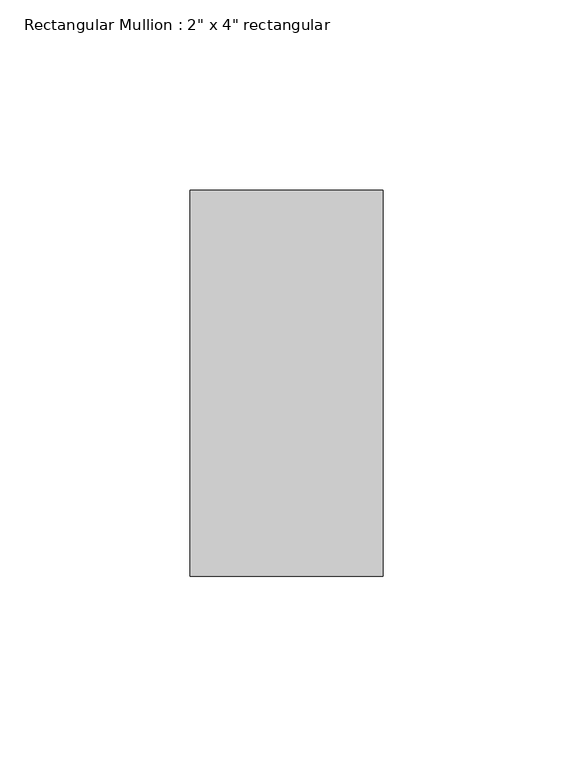
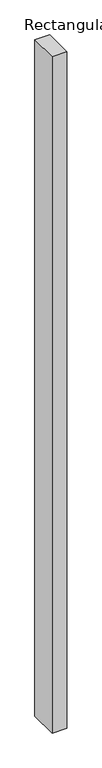
"""IFC4 building model written with IfcOpenShell, lengths in millimetres: member geometry."""

import ifcopenshell
import ifcopenshell.guid

model = None  # the IFC model being written
_history = None  # IfcOwnerHistory: only IFC2X3 demands one
_inside = {}  # id of a spatial element -> (the spatial element, [elements in it])
_under = {}  # id of a project, library or spatial element -> (it, [spatial elements below it])
_declared = {}  # id of a project -> (the project, [libraries it declares])
_typed = {}  # id of a type object -> (the type object, [elements of that type])
_made_of = {}  # id of a material, layer set ... -> (it, [elements and type objects made of it])


def new_model(schema):
    """Start an empty IFC model of exactly this schema.

    Asked for "IFC4X3", IfcOpenShell would pick the latest addendum, in which some entities
    have other attributes; the version numbers below select the first issue.
    IFC2X3 requires an IfcOwnerHistory on every rooted entity: one is made here for all.
    """
    global model, _history
    if schema == "IFC4X3":
        model = ifcopenshell.file(schema_version=(4, 3, 0, 0))
    else:
        model = ifcopenshell.file(schema=schema)
    _inside.clear()
    _under.clear()
    _declared.clear()
    _typed.clear()
    _made_of.clear()
    _history = None
    if model.schema == "IFC2X3":
        org = make("IfcOrganization", Name="unknown")
        user = make(
            "IfcPersonAndOrganization",
            ThePerson=make("IfcPerson", FamilyName="unknown"),
            TheOrganization=org,
        )
        app = make(
            "IfcApplication",
            ApplicationDeveloper=org,
            Version="unknown",
            ApplicationFullName="unknown",
            ApplicationIdentifier="unknown",
        )
        _history = make(
            "IfcOwnerHistory",
            OwningUser=user,
            OwningApplication=app,
            ChangeAction="ADDED",
            CreationDate=0,
        )
    return model


def make(cls, **values):
    """One entity of the class cls with the attributes given. An attribute that is None is left unset."""
    return model.create_entity(
        cls, **{name: value for name, value in values.items() if value is not None}
    )


def rooted(cls, **values):
    """An entity with a GlobalId (a new one), such as an element, a storey or a relation."""
    return make(cls, GlobalId=ifcopenshell.guid.new(), OwnerHistory=_history, **values)


def si_unit(unit_type, name, prefix=None):
    """IfcSIUnit, for example si_unit("LENGTHUNIT", "METRE", prefix="MILLI")."""
    return make("IfcSIUnit", UnitType=unit_type, Prefix=prefix, Name=name)


def assignment(units):
    """IfcUnitAssignment: the units of a project."""
    return None if units is None else make("IfcUnitAssignment", Units=units)


def point(xyz):
    """IfcCartesianPoint."""
    return None if xyz is None else make("IfcCartesianPoint", Coordinates=xyz)


def direction(xyz):
    """IfcDirection."""
    return None if xyz is None else make("IfcDirection", DirectionRatios=xyz)


def frame(location, z_axis=None, x_axis=None):
    """IfcAxis2Placement3D, a coordinate frame: its origin and axes. An axis left out is left unset."""
    return make(
        "IfcAxis2Placement3D",
        Location=point(location),
        Axis=direction(z_axis),
        RefDirection=direction(x_axis),
    )


def origin():
    """The frame at (0, 0, 0) with its axes left unset."""
    return frame((0.0, 0.0, 0.0))


def place(relative_to, where):
    """IfcLocalPlacement: puts the frame where relative to a parent placement (None: the world)."""
    return make(
        "IfcLocalPlacement", PlacementRelTo=relative_to, RelativePlacement=where
    )


def context(
    kind, dimensions, precision=None, world=None, true_north=None, identifier=None
):
    """IfcGeometricRepresentationContext, for example the 3D "Model" context."""
    return make(
        "IfcGeometricRepresentationContext",
        ContextIdentifier=identifier,
        ContextType=kind,
        CoordinateSpaceDimension=dimensions,
        Precision=precision,
        WorldCoordinateSystem=world,
        TrueNorth=true_north,
    )


def project(units=None, contexts=None):
    """IfcProject with its units and contexts."""
    return rooted(
        "IfcProject",
        Name="project",
        RepresentationContexts=contexts,
        UnitsInContext=assignment(units),
    )


def spatial(cls, under=None, at=None, **own):
    """A site, building, storey or space (cls), placed at a placement, below another one or the project."""
    s = rooted(cls, ObjectPlacement=at, **own)
    if under is not None:
        _under.setdefault(under.id(), (under, []))[1].append(s)
    return s


def polyline(points):
    """IfcPolyline through the points."""
    return make("IfcPolyline", Points=[point(p) for p in points])


def outline(outer, holes=None, kind="AREA"):
    """IfcArbitraryClosedProfileDef: a profile drawn as a closed curve; with holes, ...WithVoids."""
    if holes is None:
        return make("IfcArbitraryClosedProfileDef", ProfileType=kind, OuterCurve=outer)
    return make(
        "IfcArbitraryProfileDefWithVoids",
        ProfileType=kind,
        OuterCurve=outer,
        InnerCurves=holes,
    )


def extrude(swept, where, along, depth):
    """IfcExtrudedAreaSolid: the profile swept, set in the frame where, extruded along a direction by depth."""
    return make(
        "IfcExtrudedAreaSolid",
        SweptArea=swept,
        Position=where,
        ExtrudedDirection=direction(along),
        Depth=depth,
    )


def shape(context_of_items, identifier, shape_type, items):
    """IfcShapeRepresentation: the items that make up one representation, for example the "Body"."""
    return make(
        "IfcShapeRepresentation",
        ContextOfItems=context_of_items,
        RepresentationIdentifier=identifier,
        RepresentationType=shape_type,
        Items=items,
    )


def source(mapping_origin, context_of_items, identifier, shape_type, items):
    """IfcRepresentationMap: a shape defined once, which mapped items show again and again."""
    return make(
        "IfcRepresentationMap",
        MappingOrigin=mapping_origin,
        MappedRepresentation=shape(context_of_items, identifier, shape_type, items),
    )


def transform(
    local_origin,
    x_axis=None,
    y_axis=None,
    z_axis=None,
    scale=None,
    scale2=None,
    scale3=None,
    uniform=True,
):
    """IfcCartesianTransformationOperator3D, or its non-uniform kind. x_axis, y_axis, z_axis: its Axis1, 2, 3."""
    if uniform:
        return make(
            "IfcCartesianTransformationOperator3D",
            Axis1=direction(x_axis),
            Axis2=direction(y_axis),
            LocalOrigin=point(local_origin),
            Scale=scale,
            Axis3=direction(z_axis),
        )
    return make(
        "IfcCartesianTransformationOperator3DnonUniform",
        Axis1=direction(x_axis),
        Axis2=direction(y_axis),
        LocalOrigin=point(local_origin),
        Scale=scale,
        Axis3=direction(z_axis),
        Scale2=scale2,
        Scale3=scale3,
    )


def mapped(mapping_source, mapping_target):
    """IfcMappedItem: shows the shape of a source again, moved by a transform."""
    return make(
        "IfcMappedItem", MappingSource=mapping_source, MappingTarget=mapping_target
    )


def made_of(thing, what):
    """Note that an element or type object is made of a material, layer set ...; save() writes the relation."""
    if what is not None:
        _made_of.setdefault(what.id(), (what, []))[1].append(thing)
    return thing


def element(
    cls,
    number,
    at=None,
    inside=None,
    cuts=None,
    type_object=None,
    material=None,
    context=None,
    identifier="Body",
    shape_type=None,
    held_by="IfcProductDefinitionShape",
    body=None,
    shapes=None,
    **own,
):
    """One element of the class cls, such as IfcWall. Its Tag is "e" and its number.

    at: its placement. inside: the storey or other place that contains it. cuts: it is an
    opening in that element (IfcRelVoidsElement). A single representation is given by context,
    identifier, shape_type and body (its items); several are given by shapes. held_by: the class
    of the entity that holds the representations. save() writes the other relations.
    """
    e = rooted(cls, Tag="e%d" % number, ObjectPlacement=at, **own)
    if body is not None:
        shapes = [shape(context, identifier, shape_type, body)]
    if shapes is not None:
        e.Representation = make(held_by, Representations=shapes)
    if inside is not None:
        _inside.setdefault(inside.id(), (inside, []))[1].append(e)
    if cuts is not None:
        rooted(
            "IfcRelVoidsElement", RelatingBuildingElement=cuts, RelatedOpeningElement=e
        )
    if type_object is not None:
        _typed.setdefault(type_object.id(), (type_object, []))[1].append(e)
    return made_of(e, material)


def aggregate(whole, parts):
    """IfcRelAggregates: a whole, such as a stair, and the parts it consists of."""
    return rooted("IfcRelAggregates", RelatingObject=whole, RelatedObjects=parts)


def save(model, path):
    """Write the relations noted so far, then the file.

    IfcRelAggregates (storeys below a building ...), IfcRelContainedInSpatialStructure (elements
    in a storey), IfcRelDefinesByType, IfcRelAssociatesMaterial and IfcRelDeclares: one each for
    every whole, place, type object, material and project.
    """
    for whole, parts in _under.values():
        aggregate(whole, parts)
    for where, things in _inside.values():
        rooted(
            "IfcRelContainedInSpatialStructure",
            RelatedElements=things,
            RelatingStructure=where,
        )
    for kind, things in _typed.values():
        rooted("IfcRelDefinesByType", RelatedObjects=things, RelatingType=kind)
    for what, things in _made_of.values():
        rooted("IfcRelAssociatesMaterial", RelatedObjects=things, RelatingMaterial=what)
    for by, libraries in _declared.values():
        rooted("IfcRelDeclares", RelatingContext=by, RelatedDefinitions=libraries)
    model.write(path)


def member_5422db9a(model_context):
    return source(origin(), model_context, "Body", "SweptSolid", [
        extrude(outline(polyline([(25.4, 50.8), (25.4, -50.8), (-25.4, -50.8), (-25.4, 50.8), (25.4, 50.8)])), frame((0.0, 0.0, -2438.4), z_axis=(0.0, 0.0, 1.0), x_axis=(1.0, 0.0, 0.0)), (0.0, 0.0, 1.0), 2438.4),
    ])


if __name__ == "__main__":
    model = new_model("IFC4")
    model_context = context("Model", 3, world=origin())
    ifc_project = project(units=[si_unit("LENGTHUNIT", "METRE", prefix="MILLI")], contexts=[model_context])
    site = spatial("IfcSite", under=ifc_project)
    building = spatial("IfcBuilding", under=site)
    placement = place(None, origin())
    member_shape = member_5422db9a(model_context)
    element("IfcMember", 1, ObjectType="Rectangular Mullion : 2\" x 4\" rectangular", at=placement, inside=building, context=model_context, shape_type="MappedRepresentation", body=[
        mapped(member_shape, transform((0.0, 0.0, 0.0), x_axis=(1.0, 0.0, 0.0), y_axis=(0.0, 1.0, 0.0), z_axis=(0.0, 0.0, 1.0))),
    ])
    save(model, "model.ifc")

# Revit data of these elements
# Type "Rectangular Mullion : 2\" x 4\" rectangular"
#   built-in parameter 1007304 = 0.333333 (stored number, unit not read)
#   built-in parameter 1007301 = 0.0833333 (stored number, unit not read)
#   built-in parameter 1007300 = 0.0833333 (stored number, unit not read)
